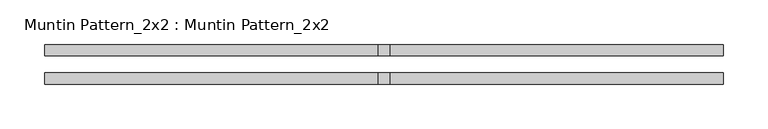
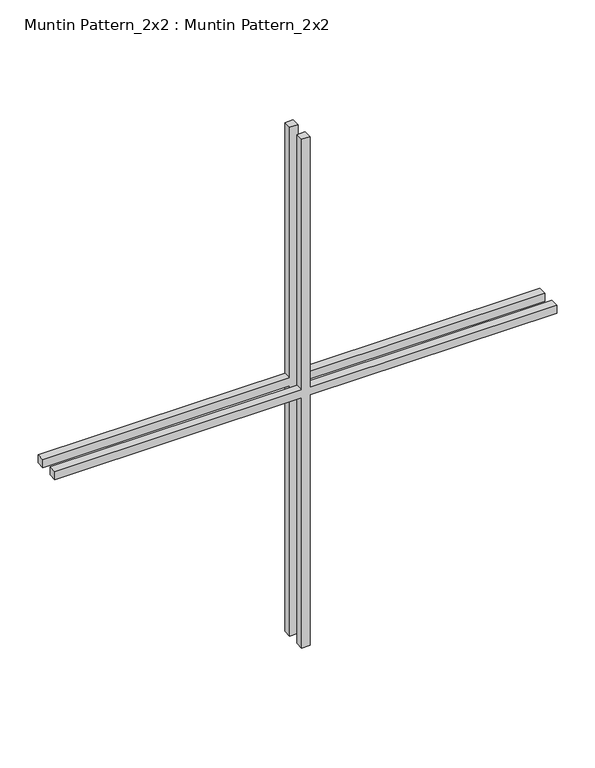
"""IFC4 building model written with IfcOpenShell, lengths in millimetres: proxy geometry, Muntin Pattern_2x2 : Muntin Pattern_2x2."""

from ifc_helpers import new_model, si_unit, frame, origin, place, context, project, spatial, polyline, outline, extrude, source, transform, mapped, element, save


def muntin_pattern_2x2_muntin_pattern_2x2_f23c1782(model_context):
    return source(origin(), model_context, "Body", "SweptSolid", [
        extrude(outline(polyline([(414.3375, -6.35), (414.3375, -381.0), (401.6375, -381.0), (401.6375, -6.35), (0.0, -6.35), (0.0, 6.35), (401.6375, 6.35), (401.6375, 381.0), (414.3375, 381.0), (414.3375, 6.35), (815.975, 6.35), (815.975, -6.35), (414.3375, -6.35)])), frame((0.0, 9.525, 0.0), z_axis=(0.0, 1.0, 0.0), x_axis=(0.0, 0.0, 1.0)), (0.0, 0.0, 1.0), 12.7),
        extrude(outline(polyline([(414.3375, -6.35), (414.3375, -381.0), (401.6375, -381.0), (401.6375, -6.35), (0.0, -6.35), (0.0, 6.35), (401.6375, 6.35), (401.6375, 381.0), (414.3375, 381.0), (414.3375, 6.35), (815.975, 6.35), (815.975, -6.35), (414.3375, -6.35)])), frame((0.0, -22.225, 0.0), z_axis=(0.0, 1.0, 0.0), x_axis=(0.0, 0.0, 1.0)), (0.0, 0.0, 1.0), 12.7),
    ])


if __name__ == "__main__":
    model = new_model("IFC4")
    model_context = context("Model", 3, world=origin())
    ifc_project = project(units=[si_unit("LENGTHUNIT", "METRE", prefix="MILLI")], contexts=[model_context])
    site = spatial("IfcSite", under=ifc_project)
    building = spatial("IfcBuilding", under=site)
    placement = place(None, origin())
    muntin_pattern_2x2_muntin_pattern_2x2_shape = muntin_pattern_2x2_muntin_pattern_2x2_f23c1782(model_context)
    element("IfcBuildingElementProxy", 1, Name="Muntin Pattern_2x2 : Muntin Pattern_2x2", ObjectType="Muntin Pattern_2x2 : Muntin Pattern_2x2", at=placement, inside=building, context=model_context, shape_type="MappedRepresentation", body=[
        mapped(muntin_pattern_2x2_muntin_pattern_2x2_shape, transform((0.0, 0.0, 0.0), x_axis=(1.0, 0.0, 0.0), y_axis=(0.0, 1.0, 0.0), z_axis=(0.0, 0.0, 1.0))),
    ])
    save(model, "model.ifc")

# Revit data of these elements
# Type "Muntin Pattern_2x2 : Muntin Pattern_2x2"
#   Width [instance default] = 4' - 0"
#   Thickness = 0' - 0 1/2"
#   Height [instance default] = 4' - 0"
#   Distance = 0' - 0 3/4"
#   Interior Material [instance default] = none
#   Exterior Material [instance default] = none
#   Default Elevation = 0
# Element 1 (IfcBuildingElementProxy, "Muntin Pattern_2x2 : Muntin Pattern_2x2")
#   Width = 2' - 6"
#   Height = 2' - 8 1/8"
#   Interior Material = Wood - Stained
#   Exterior Material = Clad - White
#   Materials on its faces: "Clad - White", "Wood - Stained"
# Materials
#   "Clad - White": class "Wood", colour RGB 242 242 238, transparency 0, Cost = 0
#   "Wood - Stained": class "Wood", colour RGB 224 178 126, transparency 0, Cost = 0
